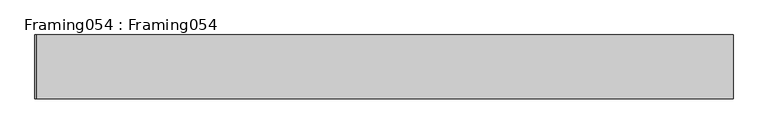
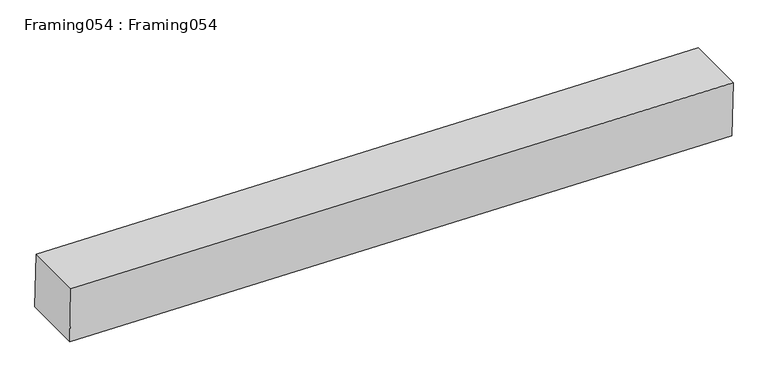
"""IFC4 building model written with IfcOpenShell, lengths in millimetres: proxy geometry, Framing054 : Framing054."""

from ifc_helpers import new_model, si_unit, frame, origin, place, context, project, spatial, polyline, outline, extrude, source, transform, mapped, element, save


def framing054_framing054_3a2aaee8(model_context):
    return source(origin(), model_context, "Body", "SweptSolid", [
        extrude(outline(polyline([(0.0, -1668.6155273), (0.0, 0.0), (152.4, 0.0), (152.4, -1668.6155273), (0.0, -1668.6155273)])), frame((-7168.279202, 9829.7531721, 39962.9678774), z_axis=(0.02089660640339769, 0.0, 0.9997816420803202), x_axis=(0.0, 1.0, 0.0)), (0.0, 0.0, 1.0), 139.7),
    ])


if __name__ == "__main__":
    model = new_model("IFC4")
    model_context = context("Model", 3, world=origin())
    ifc_project = project(units=[si_unit("LENGTHUNIT", "METRE", prefix="MILLI")], contexts=[model_context])
    site = spatial("IfcSite", under=ifc_project)
    building = spatial("IfcBuilding", under=site)
    placement = place(None, origin())
    framing054_framing054_shape = framing054_framing054_3a2aaee8(model_context)
    element("IfcBuildingElementProxy", 1, Name="Framing054 : Framing054", ObjectType="Framing054 : Framing054", at=placement, inside=building, context=model_context, shape_type="MappedRepresentation", body=[
        mapped(framing054_framing054_shape, transform((0.0, 0.0, 0.0), x_axis=(1.0, 0.0, 0.0), y_axis=(0.0, 1.0, 0.0), z_axis=(0.0, 0.0, 1.0))),
    ])
    save(model, "model.ifc")

# Revit data of these elements
# Type "Framing054 : Framing054"
#   NameOverride = "Framing054"
# Element 1 (IfcBuildingElementProxy, "Framing054 : Framing054")
#   Materials on its faces: "TAPERED 2X SLEEPERS - SLOPED TO DRAIN"
# Materials
#   "TAPERED 2X SLEEPERS - SLOPED TO DRAIN": class "Unassigned", colour RGB 234 198 178, transparency 0
